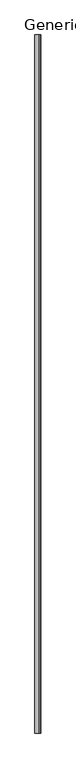
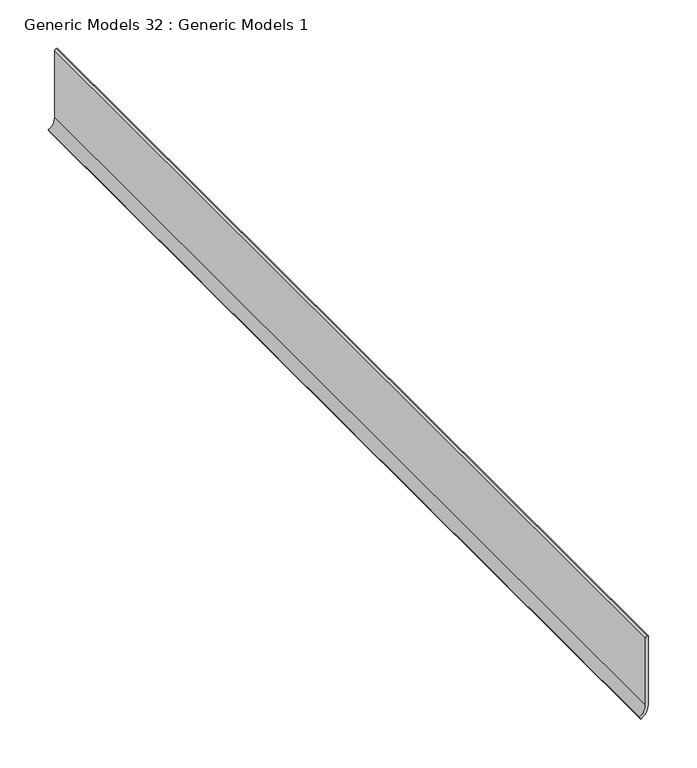
"""IFC4 building model written with IfcOpenShell, lengths in millimetres: proxy geometry, Generic Models 32 : Generic Models 1."""

import ifcopenshell
import ifcopenshell.guid

model = None  # the IFC model being written
_history = None  # IfcOwnerHistory: only IFC2X3 demands one
_inside = {}  # id of a spatial element -> (the spatial element, [elements in it])
_under = {}  # id of a project, library or spatial element -> (it, [spatial elements below it])
_declared = {}  # id of a project -> (the project, [libraries it declares])
_typed = {}  # id of a type object -> (the type object, [elements of that type])
_made_of = {}  # id of a material, layer set ... -> (it, [elements and type objects made of it])


def new_model(schema):
    """Start an empty IFC model of exactly this schema.

    Asked for "IFC4X3", IfcOpenShell would pick the latest addendum, in which some entities
    have other attributes; the version numbers below select the first issue.
    IFC2X3 requires an IfcOwnerHistory on every rooted entity: one is made here for all.
    """
    global model, _history
    if schema == "IFC4X3":
        model = ifcopenshell.file(schema_version=(4, 3, 0, 0))
    else:
        model = ifcopenshell.file(schema=schema)
    _inside.clear()
    _under.clear()
    _declared.clear()
    _typed.clear()
    _made_of.clear()
    _history = None
    if model.schema == "IFC2X3":
        org = make("IfcOrganization", Name="unknown")
        user = make(
            "IfcPersonAndOrganization",
            ThePerson=make("IfcPerson", FamilyName="unknown"),
            TheOrganization=org,
        )
        app = make(
            "IfcApplication",
            ApplicationDeveloper=org,
            Version="unknown",
            ApplicationFullName="unknown",
            ApplicationIdentifier="unknown",
        )
        _history = make(
            "IfcOwnerHistory",
            OwningUser=user,
            OwningApplication=app,
            ChangeAction="ADDED",
            CreationDate=0,
        )
    return model


def make(cls, **values):
    """One entity of the class cls with the attributes given. An attribute that is None is left unset."""
    return model.create_entity(
        cls, **{name: value for name, value in values.items() if value is not None}
    )


def rooted(cls, **values):
    """An entity with a GlobalId (a new one), such as an element, a storey or a relation."""
    return make(cls, GlobalId=ifcopenshell.guid.new(), OwnerHistory=_history, **values)


def si_unit(unit_type, name, prefix=None):
    """IfcSIUnit, for example si_unit("LENGTHUNIT", "METRE", prefix="MILLI")."""
    return make("IfcSIUnit", UnitType=unit_type, Prefix=prefix, Name=name)


def assignment(units):
    """IfcUnitAssignment: the units of a project."""
    return None if units is None else make("IfcUnitAssignment", Units=units)


def point(xyz):
    """IfcCartesianPoint."""
    return None if xyz is None else make("IfcCartesianPoint", Coordinates=xyz)


def direction(xyz):
    """IfcDirection."""
    return None if xyz is None else make("IfcDirection", DirectionRatios=xyz)


def frame(location, z_axis=None, x_axis=None):
    """IfcAxis2Placement3D, a coordinate frame: its origin and axes. An axis left out is left unset."""
    return make(
        "IfcAxis2Placement3D",
        Location=point(location),
        Axis=direction(z_axis),
        RefDirection=direction(x_axis),
    )


def frame_2d(location, x_axis=None):
    """IfcAxis2Placement2D, a coordinate frame in the plane: its origin and x axis."""
    return make(
        "IfcAxis2Placement2D", Location=point(location), RefDirection=direction(x_axis)
    )


def origin():
    """The frame at (0, 0, 0) with its axes left unset."""
    return frame((0.0, 0.0, 0.0))


def place(relative_to, where):
    """IfcLocalPlacement: puts the frame where relative to a parent placement (None: the world)."""
    return make(
        "IfcLocalPlacement", PlacementRelTo=relative_to, RelativePlacement=where
    )


def context(
    kind, dimensions, precision=None, world=None, true_north=None, identifier=None
):
    """IfcGeometricRepresentationContext, for example the 3D "Model" context."""
    return make(
        "IfcGeometricRepresentationContext",
        ContextIdentifier=identifier,
        ContextType=kind,
        CoordinateSpaceDimension=dimensions,
        Precision=precision,
        WorldCoordinateSystem=world,
        TrueNorth=true_north,
    )


def project(units=None, contexts=None):
    """IfcProject with its units and contexts."""
    return rooted(
        "IfcProject",
        Name="project",
        RepresentationContexts=contexts,
        UnitsInContext=assignment(units),
    )


def spatial(cls, under=None, at=None, **own):
    """A site, building, storey or space (cls), placed at a placement, below another one or the project."""
    s = rooted(cls, ObjectPlacement=at, **own)
    if under is not None:
        _under.setdefault(under.id(), (under, []))[1].append(s)
    return s


def polyline(points):
    """IfcPolyline through the points."""
    return make("IfcPolyline", Points=[point(p) for p in points])


def circle_curve(where, radius):
    """IfcCircle in the frame where."""
    return make("IfcCircle", Position=where, Radius=radius)


def trimmed(basis, trim1, trim2, sense, master):
    """IfcTrimmedCurve: the piece of a basis curve between two trims."""
    return make(
        "IfcTrimmedCurve",
        BasisCurve=basis,
        Trim1=trim1,
        Trim2=trim2,
        SenseAgreement=sense,
        MasterRepresentation=master,
    )


def segment(curve, same_sense, transition):
    """IfcCompositeCurveSegment."""
    return make(
        "IfcCompositeCurveSegment",
        Transition=transition,
        SameSense=same_sense,
        ParentCurve=curve,
    )


def composite_curve(segments, self_intersect=None):
    """IfcCompositeCurve: segments joined end to end."""
    return make("IfcCompositeCurve", Segments=segments, SelfIntersect=self_intersect)


def outline(outer, holes=None, kind="AREA"):
    """IfcArbitraryClosedProfileDef: a profile drawn as a closed curve; with holes, ...WithVoids."""
    if holes is None:
        return make("IfcArbitraryClosedProfileDef", ProfileType=kind, OuterCurve=outer)
    return make(
        "IfcArbitraryProfileDefWithVoids",
        ProfileType=kind,
        OuterCurve=outer,
        InnerCurves=holes,
    )


def extrude(swept, where, along, depth):
    """IfcExtrudedAreaSolid: the profile swept, set in the frame where, extruded along a direction by depth."""
    return make(
        "IfcExtrudedAreaSolid",
        SweptArea=swept,
        Position=where,
        ExtrudedDirection=direction(along),
        Depth=depth,
    )


def shape(context_of_items, identifier, shape_type, items):
    """IfcShapeRepresentation: the items that make up one representation, for example the "Body"."""
    return make(
        "IfcShapeRepresentation",
        ContextOfItems=context_of_items,
        RepresentationIdentifier=identifier,
        RepresentationType=shape_type,
        Items=items,
    )


def source(mapping_origin, context_of_items, identifier, shape_type, items):
    """IfcRepresentationMap: a shape defined once, which mapped items show again and again."""
    return make(
        "IfcRepresentationMap",
        MappingOrigin=mapping_origin,
        MappedRepresentation=shape(context_of_items, identifier, shape_type, items),
    )


def transform(
    local_origin,
    x_axis=None,
    y_axis=None,
    z_axis=None,
    scale=None,
    scale2=None,
    scale3=None,
    uniform=True,
):
    """IfcCartesianTransformationOperator3D, or its non-uniform kind. x_axis, y_axis, z_axis: its Axis1, 2, 3."""
    if uniform:
        return make(
            "IfcCartesianTransformationOperator3D",
            Axis1=direction(x_axis),
            Axis2=direction(y_axis),
            LocalOrigin=point(local_origin),
            Scale=scale,
            Axis3=direction(z_axis),
        )
    return make(
        "IfcCartesianTransformationOperator3DnonUniform",
        Axis1=direction(x_axis),
        Axis2=direction(y_axis),
        LocalOrigin=point(local_origin),
        Scale=scale,
        Axis3=direction(z_axis),
        Scale2=scale2,
        Scale3=scale3,
    )


def mapped(mapping_source, mapping_target):
    """IfcMappedItem: shows the shape of a source again, moved by a transform."""
    return make(
        "IfcMappedItem", MappingSource=mapping_source, MappingTarget=mapping_target
    )


def made_of(thing, what):
    """Note that an element or type object is made of a material, layer set ...; save() writes the relation."""
    if what is not None:
        _made_of.setdefault(what.id(), (what, []))[1].append(thing)
    return thing


def element(
    cls,
    number,
    at=None,
    inside=None,
    cuts=None,
    type_object=None,
    material=None,
    context=None,
    identifier="Body",
    shape_type=None,
    held_by="IfcProductDefinitionShape",
    body=None,
    shapes=None,
    **own,
):
    """One element of the class cls, such as IfcWall. Its Tag is "e" and its number.

    at: its placement. inside: the storey or other place that contains it. cuts: it is an
    opening in that element (IfcRelVoidsElement). A single representation is given by context,
    identifier, shape_type and body (its items); several are given by shapes. held_by: the class
    of the entity that holds the representations. save() writes the other relations.
    """
    e = rooted(cls, Tag="e%d" % number, ObjectPlacement=at, **own)
    if body is not None:
        shapes = [shape(context, identifier, shape_type, body)]
    if shapes is not None:
        e.Representation = make(held_by, Representations=shapes)
    if inside is not None:
        _inside.setdefault(inside.id(), (inside, []))[1].append(e)
    if cuts is not None:
        rooted(
            "IfcRelVoidsElement", RelatingBuildingElement=cuts, RelatedOpeningElement=e
        )
    if type_object is not None:
        _typed.setdefault(type_object.id(), (type_object, []))[1].append(e)
    return made_of(e, material)


def aggregate(whole, parts):
    """IfcRelAggregates: a whole, such as a stair, and the parts it consists of."""
    return rooted("IfcRelAggregates", RelatingObject=whole, RelatedObjects=parts)


def save(model, path):
    """Write the relations noted so far, then the file.

    IfcRelAggregates (storeys below a building ...), IfcRelContainedInSpatialStructure (elements
    in a storey), IfcRelDefinesByType, IfcRelAssociatesMaterial and IfcRelDeclares: one each for
    every whole, place, type object, material and project.
    """
    for whole, parts in _under.values():
        aggregate(whole, parts)
    for where, things in _inside.values():
        rooted(
            "IfcRelContainedInSpatialStructure",
            RelatedElements=things,
            RelatingStructure=where,
        )
    for kind, things in _typed.values():
        rooted("IfcRelDefinesByType", RelatedObjects=things, RelatingType=kind)
    for what, things in _made_of.values():
        rooted("IfcRelAssociatesMaterial", RelatedObjects=things, RelatingMaterial=what)
    for by, libraries in _declared.values():
        rooted("IfcRelDeclares", RelatingContext=by, RelatedDefinitions=libraries)
    model.write(path)


def generic_models_32_generic_models_1_fdd6cadd(model_context):
    return source(origin(), model_context, "Body", "SweptSolid", [
        extrude(outline(composite_curve([segment(polyline([(73.749588, 48367.3939813), (73.749588, 48366.3057831)]), True, "CONTINUOUS"), segment(trimmed(circle_curve(frame_2d((71.6627862, 48366.3057831)), 2.0868018), [point((73.749588, 48366.3057831))], [point((71.6627862, 48364.2189813))], False, "CARTESIAN"), True, "CONTINUOUS"), segment(polyline([(71.6627862, 48364.2189813), (-12.4007813, 48364.2189813)]), True, "CONTINUOUS"), segment(trimmed(circle_curve(frame_2d((-12.4007813, 48349.5542845)), 14.6646968), [point((-12.4007813, 48364.2189813))], [point((-25.1007813, 48356.8866329))], True, "CARTESIAN"), True, "CONTINUOUS"), segment(polyline([(-25.1007813, 48356.8866329), (-27.850412, 48358.4741329)]), True, "CONTINUOUS"), segment(trimmed(circle_curve(frame_2d((-12.4007813, 48349.5542845)), 17.8396968), [point((-27.850412, 48358.4741329))], [point((-12.4007813, 48367.3939813))], False, "CARTESIAN"), True, "CONTINUOUS"), segment(polyline([(-12.4007813, 48367.3939813), (73.749588, 48367.3939813)]), True, "CONTINUOUS")], self_intersect=False)), frame((0.0, 0.0, 0.0), z_axis=(0.0, 1.0, 0.0), x_axis=(0.0, 0.0, 1.0)), (0.0, 0.0, 1.0), 1219.2),
    ])


if __name__ == "__main__":
    model = new_model("IFC4")
    model_context = context("Model", 3, world=origin())
    ifc_project = project(units=[si_unit("LENGTHUNIT", "METRE", prefix="MILLI")], contexts=[model_context])
    site = spatial("IfcSite", under=ifc_project)
    building = spatial("IfcBuilding", under=site)
    placement = place(None, origin())
    generic_models_32_generic_models_1_shape = generic_models_32_generic_models_1_fdd6cadd(model_context)
    element("IfcBuildingElementProxy", 1, Name="Generic Models 32 : Generic Models 1", ObjectType="Generic Models 32 : Generic Models 1", at=placement, inside=building, context=model_context, shape_type="MappedRepresentation", body=[
        mapped(generic_models_32_generic_models_1_shape, transform((0.0, 0.0, 0.0), x_axis=(1.0, 0.0, 0.0), y_axis=(0.0, 1.0, 0.0), z_axis=(0.0, 0.0, 1.0))),
    ])
    save(model, "model.ifc")

# Revit data of these elements
# Element 1 (IfcBuildingElementProxy, "Generic Models 32 : Generic Models 1")
#   Materials on its faces: "BASE AS SCHEDULED"
# Materials
#   "BASE AS SCHEDULED": class "Generic", colour RGB 120 120 120, transparency 0, Cost = 0
